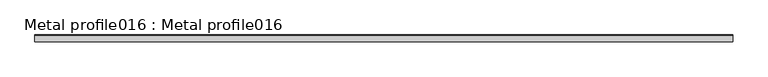
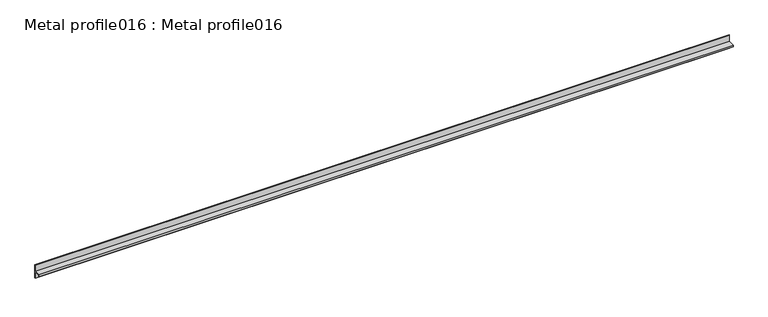
"""IFC4 building model written with IfcOpenShell, lengths in millimetres: proxy geometry, Metal profile016 : Metal profile016."""

from ifc_helpers import new_model, si_unit, frame, origin, place, context, project, spatial, polyline, outline, extrude, source, transform, mapped, element, save


def metal_profile016_metal_profile016_49e7ab77(model_context):
    return source(origin(), model_context, "Body", "SweptSolid", [
        extrude(outline(polyline([(-4433.0725368, 41040.251), (-4433.0725368, 41036.7712), (-4434.3425368, 41036.7712), (-4434.3425368, 41041.521), (-4416.1085888, 41041.521), (-4416.1085888, 41060.571), (-4414.8385888, 41060.571), (-4414.8385888, 41021.201), (-4416.1085888, 41021.201), (-4416.1085888, 41040.251), (-4433.0725368, 41040.251)])), frame((12383.0178845, 0.0, 0.0), z_axis=(1.0, 0.0, 0.0), x_axis=(0.0, 1.0, 0.0)), (0.0, 0.0, 1.0), 2000.0),
    ])


if __name__ == "__main__":
    model = new_model("IFC4")
    model_context = context("Model", 3, world=origin())
    ifc_project = project(units=[si_unit("LENGTHUNIT", "METRE", prefix="MILLI")], contexts=[model_context])
    site = spatial("IfcSite", under=ifc_project)
    building = spatial("IfcBuilding", under=site)
    placement = place(None, origin())
    metal_profile016_metal_profile016_shape = metal_profile016_metal_profile016_49e7ab77(model_context)
    element("IfcBuildingElementProxy", 1, Name="Metal profile016 : Metal profile016", ObjectType="Metal profile016 : Metal profile016", at=placement, inside=building, context=model_context, shape_type="MappedRepresentation", body=[
        mapped(metal_profile016_metal_profile016_shape, transform((0.0, 0.0, 0.0), x_axis=(1.0, 0.0, 0.0), y_axis=(0.0, 1.0, 0.0), z_axis=(0.0, 0.0, 1.0))),
    ])
    save(model, "model.ifc")

# Revit data of these elements
# Type "Metal profile016 : Metal profile016"
#   NameOverride = "Metal profile016"
# Element 1 (IfcBuildingElementProxy, "Metal profile016 : Metal profile016")
#   Materials on its faces: "16 GA. COPPER VENTED T REVEAL BEAD"
# Materials
#   "16 GA. COPPER VENTED T REVEAL BEAD": class "Unassigned", colour RGB 255 227 10, transparency 0
